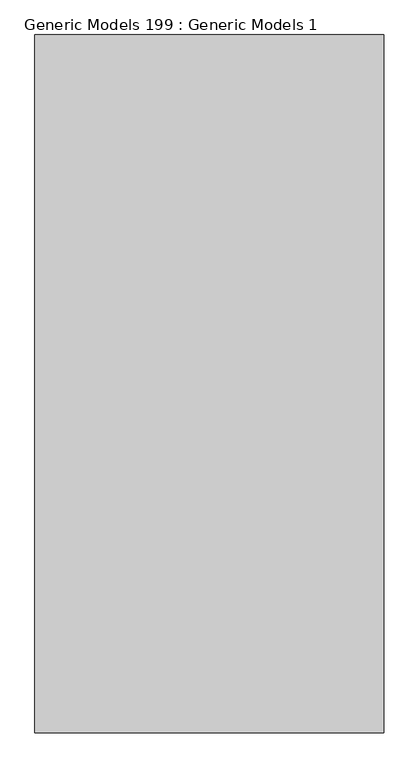
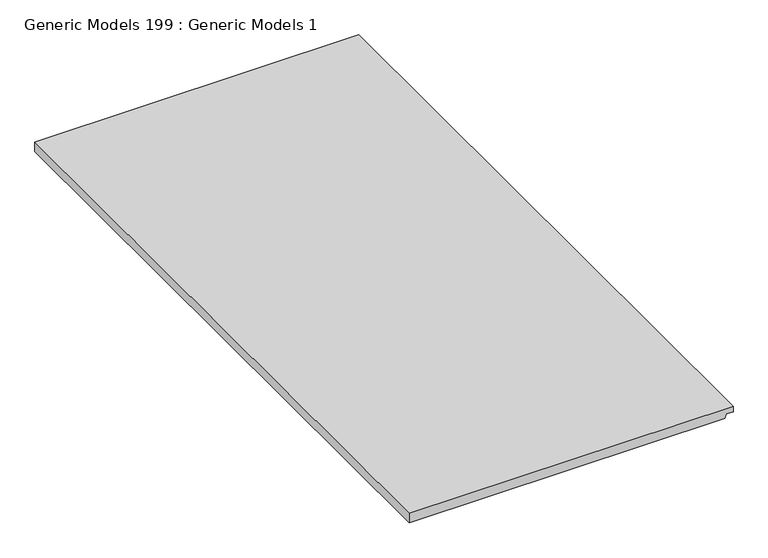
"""IFC4 building model written with IfcOpenShell, lengths in millimetres: proxy geometry, Generic Models 199 : Generic Models 1."""

import ifcopenshell
import ifcopenshell.guid

model = None  # the IFC model being written
_history = None  # IfcOwnerHistory: only IFC2X3 demands one
_inside = {}  # id of a spatial element -> (the spatial element, [elements in it])
_under = {}  # id of a project, library or spatial element -> (it, [spatial elements below it])
_declared = {}  # id of a project -> (the project, [libraries it declares])
_typed = {}  # id of a type object -> (the type object, [elements of that type])
_made_of = {}  # id of a material, layer set ... -> (it, [elements and type objects made of it])


def new_model(schema):
    """Start an empty IFC model of exactly this schema.

    Asked for "IFC4X3", IfcOpenShell would pick the latest addendum, in which some entities
    have other attributes; the version numbers below select the first issue.
    IFC2X3 requires an IfcOwnerHistory on every rooted entity: one is made here for all.
    """
    global model, _history
    if schema == "IFC4X3":
        model = ifcopenshell.file(schema_version=(4, 3, 0, 0))
    else:
        model = ifcopenshell.file(schema=schema)
    _inside.clear()
    _under.clear()
    _declared.clear()
    _typed.clear()
    _made_of.clear()
    _history = None
    if model.schema == "IFC2X3":
        org = make("IfcOrganization", Name="unknown")
        user = make(
            "IfcPersonAndOrganization",
            ThePerson=make("IfcPerson", FamilyName="unknown"),
            TheOrganization=org,
        )
        app = make(
            "IfcApplication",
            ApplicationDeveloper=org,
            Version="unknown",
            ApplicationFullName="unknown",
            ApplicationIdentifier="unknown",
        )
        _history = make(
            "IfcOwnerHistory",
            OwningUser=user,
            OwningApplication=app,
            ChangeAction="ADDED",
            CreationDate=0,
        )
    return model


def make(cls, **values):
    """One entity of the class cls with the attributes given. An attribute that is None is left unset."""
    return model.create_entity(
        cls, **{name: value for name, value in values.items() if value is not None}
    )


def rooted(cls, **values):
    """An entity with a GlobalId (a new one), such as an element, a storey or a relation."""
    return make(cls, GlobalId=ifcopenshell.guid.new(), OwnerHistory=_history, **values)


def si_unit(unit_type, name, prefix=None):
    """IfcSIUnit, for example si_unit("LENGTHUNIT", "METRE", prefix="MILLI")."""
    return make("IfcSIUnit", UnitType=unit_type, Prefix=prefix, Name=name)


def assignment(units):
    """IfcUnitAssignment: the units of a project."""
    return None if units is None else make("IfcUnitAssignment", Units=units)


def point(xyz):
    """IfcCartesianPoint."""
    return None if xyz is None else make("IfcCartesianPoint", Coordinates=xyz)


def direction(xyz):
    """IfcDirection."""
    return None if xyz is None else make("IfcDirection", DirectionRatios=xyz)


def frame(location, z_axis=None, x_axis=None):
    """IfcAxis2Placement3D, a coordinate frame: its origin and axes. An axis left out is left unset."""
    return make(
        "IfcAxis2Placement3D",
        Location=point(location),
        Axis=direction(z_axis),
        RefDirection=direction(x_axis),
    )


def origin():
    """The frame at (0, 0, 0) with its axes left unset."""
    return frame((0.0, 0.0, 0.0))


def place(relative_to, where):
    """IfcLocalPlacement: puts the frame where relative to a parent placement (None: the world)."""
    return make(
        "IfcLocalPlacement", PlacementRelTo=relative_to, RelativePlacement=where
    )


def context(
    kind, dimensions, precision=None, world=None, true_north=None, identifier=None
):
    """IfcGeometricRepresentationContext, for example the 3D "Model" context."""
    return make(
        "IfcGeometricRepresentationContext",
        ContextIdentifier=identifier,
        ContextType=kind,
        CoordinateSpaceDimension=dimensions,
        Precision=precision,
        WorldCoordinateSystem=world,
        TrueNorth=true_north,
    )


def project(units=None, contexts=None):
    """IfcProject with its units and contexts."""
    return rooted(
        "IfcProject",
        Name="project",
        RepresentationContexts=contexts,
        UnitsInContext=assignment(units),
    )


def spatial(cls, under=None, at=None, **own):
    """A site, building, storey or space (cls), placed at a placement, below another one or the project."""
    s = rooted(cls, ObjectPlacement=at, **own)
    if under is not None:
        _under.setdefault(under.id(), (under, []))[1].append(s)
    return s


def polyline(points):
    """IfcPolyline through the points."""
    return make("IfcPolyline", Points=[point(p) for p in points])


def outline(outer, holes=None, kind="AREA"):
    """IfcArbitraryClosedProfileDef: a profile drawn as a closed curve; with holes, ...WithVoids."""
    if holes is None:
        return make("IfcArbitraryClosedProfileDef", ProfileType=kind, OuterCurve=outer)
    return make(
        "IfcArbitraryProfileDefWithVoids",
        ProfileType=kind,
        OuterCurve=outer,
        InnerCurves=holes,
    )


def extrude(swept, where, along, depth):
    """IfcExtrudedAreaSolid: the profile swept, set in the frame where, extruded along a direction by depth."""
    return make(
        "IfcExtrudedAreaSolid",
        SweptArea=swept,
        Position=where,
        ExtrudedDirection=direction(along),
        Depth=depth,
    )


def shape(context_of_items, identifier, shape_type, items):
    """IfcShapeRepresentation: the items that make up one representation, for example the "Body"."""
    return make(
        "IfcShapeRepresentation",
        ContextOfItems=context_of_items,
        RepresentationIdentifier=identifier,
        RepresentationType=shape_type,
        Items=items,
    )


def source(mapping_origin, context_of_items, identifier, shape_type, items):
    """IfcRepresentationMap: a shape defined once, which mapped items show again and again."""
    return make(
        "IfcRepresentationMap",
        MappingOrigin=mapping_origin,
        MappedRepresentation=shape(context_of_items, identifier, shape_type, items),
    )


def transform(
    local_origin,
    x_axis=None,
    y_axis=None,
    z_axis=None,
    scale=None,
    scale2=None,
    scale3=None,
    uniform=True,
):
    """IfcCartesianTransformationOperator3D, or its non-uniform kind. x_axis, y_axis, z_axis: its Axis1, 2, 3."""
    if uniform:
        return make(
            "IfcCartesianTransformationOperator3D",
            Axis1=direction(x_axis),
            Axis2=direction(y_axis),
            LocalOrigin=point(local_origin),
            Scale=scale,
            Axis3=direction(z_axis),
        )
    return make(
        "IfcCartesianTransformationOperator3DnonUniform",
        Axis1=direction(x_axis),
        Axis2=direction(y_axis),
        LocalOrigin=point(local_origin),
        Scale=scale,
        Axis3=direction(z_axis),
        Scale2=scale2,
        Scale3=scale3,
    )


def mapped(mapping_source, mapping_target):
    """IfcMappedItem: shows the shape of a source again, moved by a transform."""
    return make(
        "IfcMappedItem", MappingSource=mapping_source, MappingTarget=mapping_target
    )


def made_of(thing, what):
    """Note that an element or type object is made of a material, layer set ...; save() writes the relation."""
    if what is not None:
        _made_of.setdefault(what.id(), (what, []))[1].append(thing)
    return thing


def element(
    cls,
    number,
    at=None,
    inside=None,
    cuts=None,
    type_object=None,
    material=None,
    context=None,
    identifier="Body",
    shape_type=None,
    held_by="IfcProductDefinitionShape",
    body=None,
    shapes=None,
    **own,
):
    """One element of the class cls, such as IfcWall. Its Tag is "e" and its number.

    at: its placement. inside: the storey or other place that contains it. cuts: it is an
    opening in that element (IfcRelVoidsElement). A single representation is given by context,
    identifier, shape_type and body (its items); several are given by shapes. held_by: the class
    of the entity that holds the representations. save() writes the other relations.
    """
    e = rooted(cls, Tag="e%d" % number, ObjectPlacement=at, **own)
    if body is not None:
        shapes = [shape(context, identifier, shape_type, body)]
    if shapes is not None:
        e.Representation = make(held_by, Representations=shapes)
    if inside is not None:
        _inside.setdefault(inside.id(), (inside, []))[1].append(e)
    if cuts is not None:
        rooted(
            "IfcRelVoidsElement", RelatingBuildingElement=cuts, RelatedOpeningElement=e
        )
    if type_object is not None:
        _typed.setdefault(type_object.id(), (type_object, []))[1].append(e)
    return made_of(e, material)


def aggregate(whole, parts):
    """IfcRelAggregates: a whole, such as a stair, and the parts it consists of."""
    return rooted("IfcRelAggregates", RelatingObject=whole, RelatedObjects=parts)


def save(model, path):
    """Write the relations noted so far, then the file.

    IfcRelAggregates (storeys below a building ...), IfcRelContainedInSpatialStructure (elements
    in a storey), IfcRelDefinesByType, IfcRelAssociatesMaterial and IfcRelDeclares: one each for
    every whole, place, type object, material and project.
    """
    for whole, parts in _under.values():
        aggregate(whole, parts)
    for where, things in _inside.values():
        rooted(
            "IfcRelContainedInSpatialStructure",
            RelatedElements=things,
            RelatingStructure=where,
        )
    for kind, things in _typed.values():
        rooted("IfcRelDefinesByType", RelatedObjects=things, RelatingType=kind)
    for what, things in _made_of.values():
        rooted("IfcRelAssociatesMaterial", RelatedObjects=things, RelatingMaterial=what)
    for by, libraries in _declared.values():
        rooted("IfcRelDeclares", RelatingContext=by, RelatedDefinitions=libraries)
    model.write(path)


def generic_models_199_generic_models_1_e96594cc(model_context):
    return source(origin(), model_context, "Body", "SweptSolid", [
        extrude(outline(polyline([(328.8831074, 52529.0244701), (328.8831074, 51919.4244701), (309.8331074, 51919.4244701), (309.8331074, 52513.4354563), (317.7706074, 52516.3244701), (317.7706074, 52529.0244701), (328.8831074, 52529.0244701)])), frame((0.0, 0.0, 0.0), z_axis=(0.0, 1.0, 0.0), x_axis=(0.0, 0.0, 1.0)), (0.0, 0.0, 1.0), 1219.2),
    ])


if __name__ == "__main__":
    model = new_model("IFC4")
    model_context = context("Model", 3, world=origin())
    ifc_project = project(units=[si_unit("LENGTHUNIT", "METRE", prefix="MILLI")], contexts=[model_context])
    site = spatial("IfcSite", under=ifc_project)
    building = spatial("IfcBuilding", under=site)
    placement = place(None, origin())
    generic_models_199_generic_models_1_shape = generic_models_199_generic_models_1_e96594cc(model_context)
    element("IfcBuildingElementProxy", 1, Name="Generic Models 199 : Generic Models 1", ObjectType="Generic Models 199 : Generic Models 1", at=placement, inside=building, context=model_context, shape_type="MappedRepresentation", body=[
        mapped(generic_models_199_generic_models_1_shape, transform((0.0, 0.0, 0.0), x_axis=(1.0, 0.0, 0.0), y_axis=(0.0, 1.0, 0.0), z_axis=(0.0, 0.0, 1.0))),
    ])
    save(model, "model.ifc")

# Revit data of these elements
# Element 1 (IfcBuildingElementProxy, "Generic Models 199 : Generic Models 1")
#   Materials on its faces: "EXISTING ACT CEILING"
# Materials
#   "EXISTING ACT CEILING": class "Generic", colour RGB 255 255 255, transparency 0, Cost = 0
